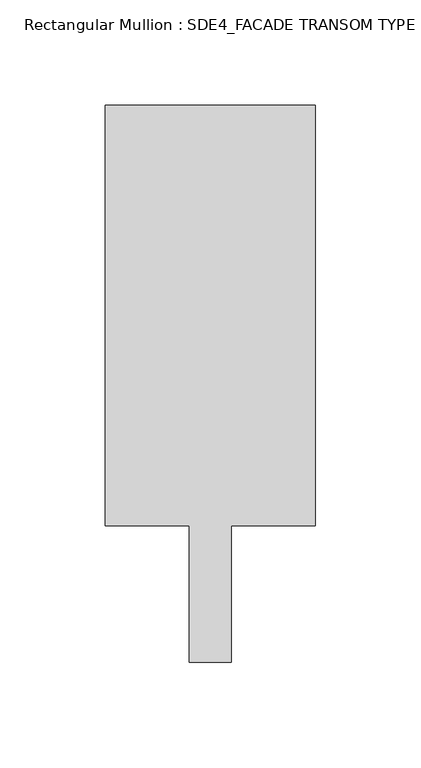
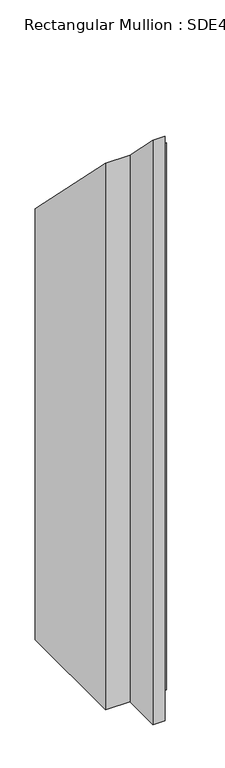
"""IFC4 building model written with IfcOpenShell, lengths in millimetres: member geometry, Rectangular Mullion : SDE4_FACADE TRANSOM TYPE 2."""

import ifcopenshell
import ifcopenshell.guid

model = None  # the IFC model being written
_history = None  # IfcOwnerHistory: only IFC2X3 demands one
_inside = {}  # id of a spatial element -> (the spatial element, [elements in it])
_under = {}  # id of a project, library or spatial element -> (it, [spatial elements below it])
_declared = {}  # id of a project -> (the project, [libraries it declares])
_typed = {}  # id of a type object -> (the type object, [elements of that type])
_made_of = {}  # id of a material, layer set ... -> (it, [elements and type objects made of it])


def new_model(schema):
    """Start an empty IFC model of exactly this schema.

    Asked for "IFC4X3", IfcOpenShell would pick the latest addendum, in which some entities
    have other attributes; the version numbers below select the first issue.
    IFC2X3 requires an IfcOwnerHistory on every rooted entity: one is made here for all.
    """
    global model, _history
    if schema == "IFC4X3":
        model = ifcopenshell.file(schema_version=(4, 3, 0, 0))
    else:
        model = ifcopenshell.file(schema=schema)
    _inside.clear()
    _under.clear()
    _declared.clear()
    _typed.clear()
    _made_of.clear()
    _history = None
    if model.schema == "IFC2X3":
        org = make("IfcOrganization", Name="unknown")
        user = make(
            "IfcPersonAndOrganization",
            ThePerson=make("IfcPerson", FamilyName="unknown"),
            TheOrganization=org,
        )
        app = make(
            "IfcApplication",
            ApplicationDeveloper=org,
            Version="unknown",
            ApplicationFullName="unknown",
            ApplicationIdentifier="unknown",
        )
        _history = make(
            "IfcOwnerHistory",
            OwningUser=user,
            OwningApplication=app,
            ChangeAction="ADDED",
            CreationDate=0,
        )
    return model


def make(cls, **values):
    """One entity of the class cls with the attributes given. An attribute that is None is left unset."""
    return model.create_entity(
        cls, **{name: value for name, value in values.items() if value is not None}
    )


def rooted(cls, **values):
    """An entity with a GlobalId (a new one), such as an element, a storey or a relation."""
    return make(cls, GlobalId=ifcopenshell.guid.new(), OwnerHistory=_history, **values)


def si_unit(unit_type, name, prefix=None):
    """IfcSIUnit, for example si_unit("LENGTHUNIT", "METRE", prefix="MILLI")."""
    return make("IfcSIUnit", UnitType=unit_type, Prefix=prefix, Name=name)


def assignment(units):
    """IfcUnitAssignment: the units of a project."""
    return None if units is None else make("IfcUnitAssignment", Units=units)


def point(xyz):
    """IfcCartesianPoint."""
    return None if xyz is None else make("IfcCartesianPoint", Coordinates=xyz)


def direction(xyz):
    """IfcDirection."""
    return None if xyz is None else make("IfcDirection", DirectionRatios=xyz)


def frame(location, z_axis=None, x_axis=None):
    """IfcAxis2Placement3D, a coordinate frame: its origin and axes. An axis left out is left unset."""
    return make(
        "IfcAxis2Placement3D",
        Location=point(location),
        Axis=direction(z_axis),
        RefDirection=direction(x_axis),
    )


def origin():
    """The frame at (0, 0, 0) with its axes left unset."""
    return frame((0.0, 0.0, 0.0))


def place(relative_to, where):
    """IfcLocalPlacement: puts the frame where relative to a parent placement (None: the world)."""
    return make(
        "IfcLocalPlacement", PlacementRelTo=relative_to, RelativePlacement=where
    )


def context(
    kind, dimensions, precision=None, world=None, true_north=None, identifier=None
):
    """IfcGeometricRepresentationContext, for example the 3D "Model" context."""
    return make(
        "IfcGeometricRepresentationContext",
        ContextIdentifier=identifier,
        ContextType=kind,
        CoordinateSpaceDimension=dimensions,
        Precision=precision,
        WorldCoordinateSystem=world,
        TrueNorth=true_north,
    )


def project(units=None, contexts=None):
    """IfcProject with its units and contexts."""
    return rooted(
        "IfcProject",
        Name="project",
        RepresentationContexts=contexts,
        UnitsInContext=assignment(units),
    )


def spatial(cls, under=None, at=None, **own):
    """A site, building, storey or space (cls), placed at a placement, below another one or the project."""
    s = rooted(cls, ObjectPlacement=at, **own)
    if under is not None:
        _under.setdefault(under.id(), (under, []))[1].append(s)
    return s


def faces_of(points, faces, orient=None, outer=None):
    """IfcFace entities. A face is a list of loops; a loop is a list of indices into points, from 0.

    orient and outer hold one flag for each loop. By default every Orientation is true, the
    first loop of a face is its IfcFaceOuterBound and the others are IfcFaceBound.
    """
    made = []
    for i, loops in enumerate(faces):
        bounds = []
        for j, loop in enumerate(loops):
            is_outer = j == 0 if outer is None else outer[i][j]
            bounds.append(
                make(
                    "IfcFaceOuterBound" if is_outer else "IfcFaceBound",
                    Bound=make("IfcPolyLoop", Polygon=[points[k] for k in loop]),
                    Orientation=True if orient is None else orient[i][j],
                )
            )
        made.append(make("IfcFace", Bounds=bounds))
    return made


def faceted_brep(points, faces, orient=None, outer=None, voids=None):
    """IfcFacetedBrep: a solid bounded by flat faces; with voids (closed shells), ...WithVoids."""
    shared = [point(p) for p in points]
    hull = make("IfcClosedShell", CfsFaces=faces_of(shared, faces, orient, outer))
    if voids is None:
        return make("IfcFacetedBrep", Outer=hull)
    return make(
        "IfcFacetedBrepWithVoids",
        Outer=hull,
        Voids=[
            make(cls, CfsFaces=faces_of(shared, fs, o, b)) for cls, fs, o, b in voids
        ],
    )


def shape(context_of_items, identifier, shape_type, items):
    """IfcShapeRepresentation: the items that make up one representation, for example the "Body"."""
    return make(
        "IfcShapeRepresentation",
        ContextOfItems=context_of_items,
        RepresentationIdentifier=identifier,
        RepresentationType=shape_type,
        Items=items,
    )


def source(mapping_origin, context_of_items, identifier, shape_type, items):
    """IfcRepresentationMap: a shape defined once, which mapped items show again and again."""
    return make(
        "IfcRepresentationMap",
        MappingOrigin=mapping_origin,
        MappedRepresentation=shape(context_of_items, identifier, shape_type, items),
    )


def transform(
    local_origin,
    x_axis=None,
    y_axis=None,
    z_axis=None,
    scale=None,
    scale2=None,
    scale3=None,
    uniform=True,
):
    """IfcCartesianTransformationOperator3D, or its non-uniform kind. x_axis, y_axis, z_axis: its Axis1, 2, 3."""
    if uniform:
        return make(
            "IfcCartesianTransformationOperator3D",
            Axis1=direction(x_axis),
            Axis2=direction(y_axis),
            LocalOrigin=point(local_origin),
            Scale=scale,
            Axis3=direction(z_axis),
        )
    return make(
        "IfcCartesianTransformationOperator3DnonUniform",
        Axis1=direction(x_axis),
        Axis2=direction(y_axis),
        LocalOrigin=point(local_origin),
        Scale=scale,
        Axis3=direction(z_axis),
        Scale2=scale2,
        Scale3=scale3,
    )


def mapped(mapping_source, mapping_target):
    """IfcMappedItem: shows the shape of a source again, moved by a transform."""
    return make(
        "IfcMappedItem", MappingSource=mapping_source, MappingTarget=mapping_target
    )


def made_of(thing, what):
    """Note that an element or type object is made of a material, layer set ...; save() writes the relation."""
    if what is not None:
        _made_of.setdefault(what.id(), (what, []))[1].append(thing)
    return thing


def element(
    cls,
    number,
    at=None,
    inside=None,
    cuts=None,
    type_object=None,
    material=None,
    context=None,
    identifier="Body",
    shape_type=None,
    held_by="IfcProductDefinitionShape",
    body=None,
    shapes=None,
    **own,
):
    """One element of the class cls, such as IfcWall. Its Tag is "e" and its number.

    at: its placement. inside: the storey or other place that contains it. cuts: it is an
    opening in that element (IfcRelVoidsElement). A single representation is given by context,
    identifier, shape_type and body (its items); several are given by shapes. held_by: the class
    of the entity that holds the representations. save() writes the other relations.
    """
    e = rooted(cls, Tag="e%d" % number, ObjectPlacement=at, **own)
    if body is not None:
        shapes = [shape(context, identifier, shape_type, body)]
    if shapes is not None:
        e.Representation = make(held_by, Representations=shapes)
    if inside is not None:
        _inside.setdefault(inside.id(), (inside, []))[1].append(e)
    if cuts is not None:
        rooted(
            "IfcRelVoidsElement", RelatingBuildingElement=cuts, RelatedOpeningElement=e
        )
    if type_object is not None:
        _typed.setdefault(type_object.id(), (type_object, []))[1].append(e)
    return made_of(e, material)


def aggregate(whole, parts):
    """IfcRelAggregates: a whole, such as a stair, and the parts it consists of."""
    return rooted("IfcRelAggregates", RelatingObject=whole, RelatedObjects=parts)


def save(model, path):
    """Write the relations noted so far, then the file.

    IfcRelAggregates (storeys below a building ...), IfcRelContainedInSpatialStructure (elements
    in a storey), IfcRelDefinesByType, IfcRelAssociatesMaterial and IfcRelDeclares: one each for
    every whole, place, type object, material and project.
    """
    for whole, parts in _under.values():
        aggregate(whole, parts)
    for where, things in _inside.values():
        rooted(
            "IfcRelContainedInSpatialStructure",
            RelatedElements=things,
            RelatingStructure=where,
        )
    for kind, things in _typed.values():
        rooted("IfcRelDefinesByType", RelatedObjects=things, RelatingType=kind)
    for what, things in _made_of.values():
        rooted("IfcRelAssociatesMaterial", RelatedObjects=things, RelatingMaterial=what)
    for by, libraries in _declared.values():
        rooted("IfcRelDeclares", RelatingContext=by, RelatedDefinitions=libraries)
    model.write(path)


def rectangular_mullion_sde4_facade_transom_type_2_7cf2d938(model_context):
    return source(origin(), model_context, "Body", "Brep", [
        faceted_brep([(50.0, 132.5, -878.5000001), (50.0, -67.5, -878.5000001), (10.0, -67.5, -878.5000001), (10.0, -132.5, -878.5000001), (-10.0, -132.5, -878.5000001), (-10.0, -67.5, -878.5000001), (-50.0, -67.5, -878.5000001), (-50.0, 132.5, -878.5000001), (-50.0, 132.5, -132.5), (50.0, 132.5, -132.5), (-50.0, -67.5, 67.5), (-10.0, -67.5, 67.5), (-10.0, -132.5, 132.5), (10.0, -132.5, 132.5), (10.0, -67.5, 67.5), (50.0, -67.5, 67.5)], [[[0, 1, 2, 3, 4, 5, 6, 7]], [[8, 9, 0, 7]], [[10, 8, 7, 6]], [[11, 10, 6, 5]], [[12, 11, 5, 4]], [[13, 12, 4, 3]], [[14, 13, 3, 2]], [[15, 14, 2, 1]], [[9, 15, 1, 0]], [[9, 8, 10, 11, 12, 13, 14, 15]]]),
    ])


if __name__ == "__main__":
    model = new_model("IFC4")
    model_context = context("Model", 3, world=origin())
    ifc_project = project(units=[si_unit("LENGTHUNIT", "METRE", prefix="MILLI")], contexts=[model_context])
    site = spatial("IfcSite", under=ifc_project)
    building = spatial("IfcBuilding", under=site)
    placement = place(None, origin())
    rectangular_mullion_sde4_facade_transom_type_2_shape = rectangular_mullion_sde4_facade_transom_type_2_7cf2d938(model_context)
    element("IfcMember", 1, ObjectType="Rectangular Mullion : SDE4_FACADE TRANSOM TYPE 2", at=placement, inside=building, context=model_context, shape_type="MappedRepresentation", body=[
        mapped(rectangular_mullion_sde4_facade_transom_type_2_shape, transform((0.0, 0.0, 0.0), x_axis=(1.0, 0.0, 0.0), y_axis=(0.0, 1.0, 0.0), z_axis=(0.0, 0.0, 1.0))),
    ])
    save(model, "model.ifc")

# Revit data of these elements
# Type "Rectangular Mullion : SDE4_FACADE TRANSOM TYPE 2"
#   built-in parameter 1007322 = 0.869423 (stored number, unit not read)
#   built-in parameter 1007321 = 0.164042 (stored number, unit not read)
#   built-in parameter 1007320 = 0.164042 (stored number, unit not read)
